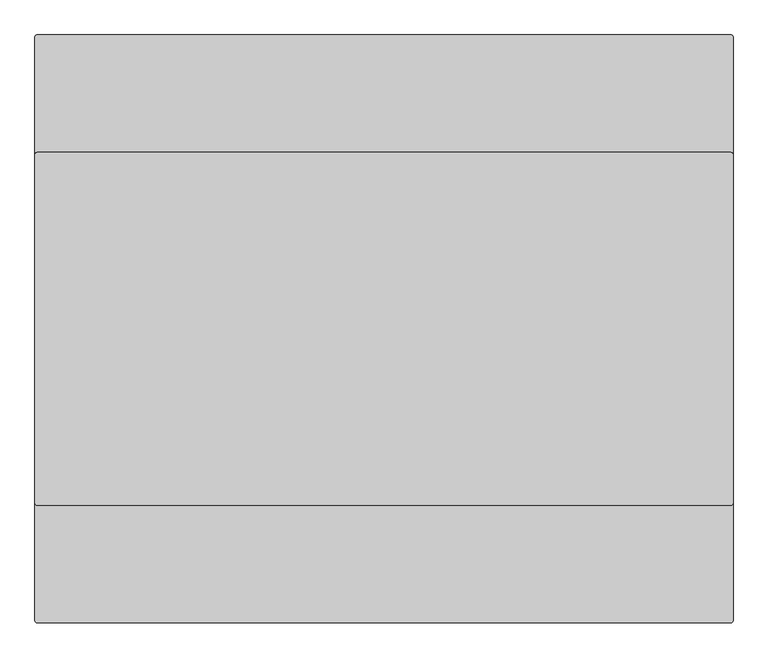
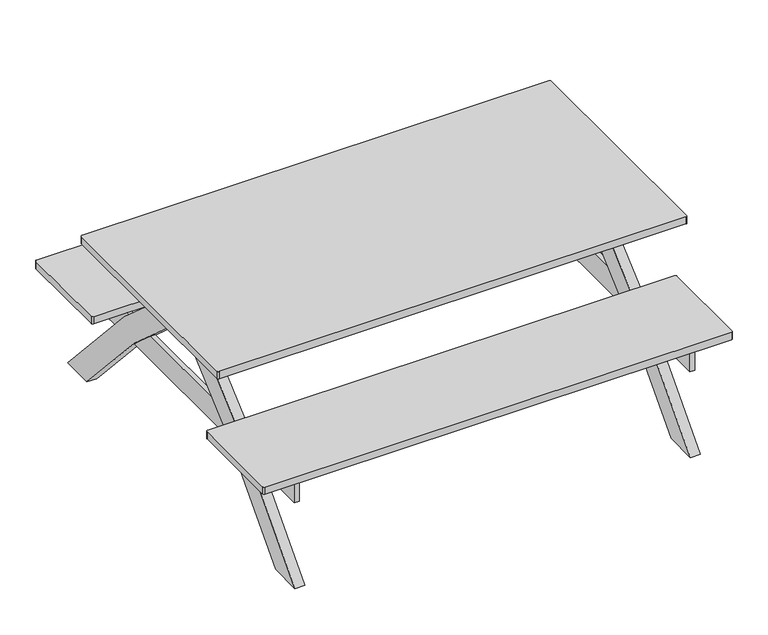
"""IFC4 building model written with IfcOpenShell, lengths in millimetres: furniture geometry, NLRS_90_FU_WPB_picknick tafel_gen_rsf : picknicktafel hout lxbxh 1900x1600x750mm."""

import ifcopenshell
import ifcopenshell.guid

model = None  # the IFC model being written
_history = None  # IfcOwnerHistory: only IFC2X3 demands one
_inside = {}  # id of a spatial element -> (the spatial element, [elements in it])
_under = {}  # id of a project, library or spatial element -> (it, [spatial elements below it])
_declared = {}  # id of a project -> (the project, [libraries it declares])
_typed = {}  # id of a type object -> (the type object, [elements of that type])
_made_of = {}  # id of a material, layer set ... -> (it, [elements and type objects made of it])


def new_model(schema):
    """Start an empty IFC model of exactly this schema.

    Asked for "IFC4X3", IfcOpenShell would pick the latest addendum, in which some entities
    have other attributes; the version numbers below select the first issue.
    IFC2X3 requires an IfcOwnerHistory on every rooted entity: one is made here for all.
    """
    global model, _history
    if schema == "IFC4X3":
        model = ifcopenshell.file(schema_version=(4, 3, 0, 0))
    else:
        model = ifcopenshell.file(schema=schema)
    _inside.clear()
    _under.clear()
    _declared.clear()
    _typed.clear()
    _made_of.clear()
    _history = None
    if model.schema == "IFC2X3":
        org = make("IfcOrganization", Name="unknown")
        user = make(
            "IfcPersonAndOrganization",
            ThePerson=make("IfcPerson", FamilyName="unknown"),
            TheOrganization=org,
        )
        app = make(
            "IfcApplication",
            ApplicationDeveloper=org,
            Version="unknown",
            ApplicationFullName="unknown",
            ApplicationIdentifier="unknown",
        )
        _history = make(
            "IfcOwnerHistory",
            OwningUser=user,
            OwningApplication=app,
            ChangeAction="ADDED",
            CreationDate=0,
        )
    return model


def make(cls, **values):
    """One entity of the class cls with the attributes given. An attribute that is None is left unset."""
    return model.create_entity(
        cls, **{name: value for name, value in values.items() if value is not None}
    )


def rooted(cls, **values):
    """An entity with a GlobalId (a new one), such as an element, a storey or a relation."""
    return make(cls, GlobalId=ifcopenshell.guid.new(), OwnerHistory=_history, **values)


def si_unit(unit_type, name, prefix=None):
    """IfcSIUnit, for example si_unit("LENGTHUNIT", "METRE", prefix="MILLI")."""
    return make("IfcSIUnit", UnitType=unit_type, Prefix=prefix, Name=name)


def assignment(units):
    """IfcUnitAssignment: the units of a project."""
    return None if units is None else make("IfcUnitAssignment", Units=units)


def point(xyz):
    """IfcCartesianPoint."""
    return None if xyz is None else make("IfcCartesianPoint", Coordinates=xyz)


def direction(xyz):
    """IfcDirection."""
    return None if xyz is None else make("IfcDirection", DirectionRatios=xyz)


def frame(location, z_axis=None, x_axis=None):
    """IfcAxis2Placement3D, a coordinate frame: its origin and axes. An axis left out is left unset."""
    return make(
        "IfcAxis2Placement3D",
        Location=point(location),
        Axis=direction(z_axis),
        RefDirection=direction(x_axis),
    )


def frame_2d(location, x_axis=None):
    """IfcAxis2Placement2D, a coordinate frame in the plane: its origin and x axis."""
    return make(
        "IfcAxis2Placement2D", Location=point(location), RefDirection=direction(x_axis)
    )


def origin():
    """The frame at (0, 0, 0) with its axes left unset."""
    return frame((0.0, 0.0, 0.0))


def place(relative_to, where):
    """IfcLocalPlacement: puts the frame where relative to a parent placement (None: the world)."""
    return make(
        "IfcLocalPlacement", PlacementRelTo=relative_to, RelativePlacement=where
    )


def context(
    kind, dimensions, precision=None, world=None, true_north=None, identifier=None
):
    """IfcGeometricRepresentationContext, for example the 3D "Model" context."""
    return make(
        "IfcGeometricRepresentationContext",
        ContextIdentifier=identifier,
        ContextType=kind,
        CoordinateSpaceDimension=dimensions,
        Precision=precision,
        WorldCoordinateSystem=world,
        TrueNorth=true_north,
    )


def project(units=None, contexts=None):
    """IfcProject with its units and contexts."""
    return rooted(
        "IfcProject",
        Name="project",
        RepresentationContexts=contexts,
        UnitsInContext=assignment(units),
    )


def spatial(cls, under=None, at=None, **own):
    """A site, building, storey or space (cls), placed at a placement, below another one or the project."""
    s = rooted(cls, ObjectPlacement=at, **own)
    if under is not None:
        _under.setdefault(under.id(), (under, []))[1].append(s)
    return s


def polyline(points):
    """IfcPolyline through the points."""
    return make("IfcPolyline", Points=[point(p) for p in points])


def circle_curve(where, radius):
    """IfcCircle in the frame where."""
    return make("IfcCircle", Position=where, Radius=radius)


def trimmed(basis, trim1, trim2, sense, master):
    """IfcTrimmedCurve: the piece of a basis curve between two trims."""
    return make(
        "IfcTrimmedCurve",
        BasisCurve=basis,
        Trim1=trim1,
        Trim2=trim2,
        SenseAgreement=sense,
        MasterRepresentation=master,
    )


def segment(curve, same_sense, transition):
    """IfcCompositeCurveSegment."""
    return make(
        "IfcCompositeCurveSegment",
        Transition=transition,
        SameSense=same_sense,
        ParentCurve=curve,
    )


def composite_curve(segments, self_intersect=None):
    """IfcCompositeCurve: segments joined end to end."""
    return make("IfcCompositeCurve", Segments=segments, SelfIntersect=self_intersect)


def outline(outer, holes=None, kind="AREA"):
    """IfcArbitraryClosedProfileDef: a profile drawn as a closed curve; with holes, ...WithVoids."""
    if holes is None:
        return make("IfcArbitraryClosedProfileDef", ProfileType=kind, OuterCurve=outer)
    return make(
        "IfcArbitraryProfileDefWithVoids",
        ProfileType=kind,
        OuterCurve=outer,
        InnerCurves=holes,
    )


def extrude(swept, where, along, depth):
    """IfcExtrudedAreaSolid: the profile swept, set in the frame where, extruded along a direction by depth."""
    return make(
        "IfcExtrudedAreaSolid",
        SweptArea=swept,
        Position=where,
        ExtrudedDirection=direction(along),
        Depth=depth,
    )


def faces_of(points, faces, orient=None, outer=None):
    """IfcFace entities. A face is a list of loops; a loop is a list of indices into points, from 0.

    orient and outer hold one flag for each loop. By default every Orientation is true, the
    first loop of a face is its IfcFaceOuterBound and the others are IfcFaceBound.
    """
    made = []
    for i, loops in enumerate(faces):
        bounds = []
        for j, loop in enumerate(loops):
            is_outer = j == 0 if outer is None else outer[i][j]
            bounds.append(
                make(
                    "IfcFaceOuterBound" if is_outer else "IfcFaceBound",
                    Bound=make("IfcPolyLoop", Polygon=[points[k] for k in loop]),
                    Orientation=True if orient is None else orient[i][j],
                )
            )
        made.append(make("IfcFace", Bounds=bounds))
    return made


def faceted_brep(points, faces, orient=None, outer=None, voids=None):
    """IfcFacetedBrep: a solid bounded by flat faces; with voids (closed shells), ...WithVoids."""
    shared = [point(p) for p in points]
    hull = make("IfcClosedShell", CfsFaces=faces_of(shared, faces, orient, outer))
    if voids is None:
        return make("IfcFacetedBrep", Outer=hull)
    return make(
        "IfcFacetedBrepWithVoids",
        Outer=hull,
        Voids=[
            make(cls, CfsFaces=faces_of(shared, fs, o, b)) for cls, fs, o, b in voids
        ],
    )


def shape(context_of_items, identifier, shape_type, items):
    """IfcShapeRepresentation: the items that make up one representation, for example the "Body"."""
    return make(
        "IfcShapeRepresentation",
        ContextOfItems=context_of_items,
        RepresentationIdentifier=identifier,
        RepresentationType=shape_type,
        Items=items,
    )


def source(mapping_origin, context_of_items, identifier, shape_type, items):
    """IfcRepresentationMap: a shape defined once, which mapped items show again and again."""
    return make(
        "IfcRepresentationMap",
        MappingOrigin=mapping_origin,
        MappedRepresentation=shape(context_of_items, identifier, shape_type, items),
    )


def transform(
    local_origin,
    x_axis=None,
    y_axis=None,
    z_axis=None,
    scale=None,
    scale2=None,
    scale3=None,
    uniform=True,
):
    """IfcCartesianTransformationOperator3D, or its non-uniform kind. x_axis, y_axis, z_axis: its Axis1, 2, 3."""
    if uniform:
        return make(
            "IfcCartesianTransformationOperator3D",
            Axis1=direction(x_axis),
            Axis2=direction(y_axis),
            LocalOrigin=point(local_origin),
            Scale=scale,
            Axis3=direction(z_axis),
        )
    return make(
        "IfcCartesianTransformationOperator3DnonUniform",
        Axis1=direction(x_axis),
        Axis2=direction(y_axis),
        LocalOrigin=point(local_origin),
        Scale=scale,
        Axis3=direction(z_axis),
        Scale2=scale2,
        Scale3=scale3,
    )


def mapped(mapping_source, mapping_target):
    """IfcMappedItem: shows the shape of a source again, moved by a transform."""
    return make(
        "IfcMappedItem", MappingSource=mapping_source, MappingTarget=mapping_target
    )


def made_of(thing, what):
    """Note that an element or type object is made of a material, layer set ...; save() writes the relation."""
    if what is not None:
        _made_of.setdefault(what.id(), (what, []))[1].append(thing)
    return thing


def element(
    cls,
    number,
    at=None,
    inside=None,
    cuts=None,
    type_object=None,
    material=None,
    context=None,
    identifier="Body",
    shape_type=None,
    held_by="IfcProductDefinitionShape",
    body=None,
    shapes=None,
    **own,
):
    """One element of the class cls, such as IfcWall. Its Tag is "e" and its number.

    at: its placement. inside: the storey or other place that contains it. cuts: it is an
    opening in that element (IfcRelVoidsElement). A single representation is given by context,
    identifier, shape_type and body (its items); several are given by shapes. held_by: the class
    of the entity that holds the representations. save() writes the other relations.
    """
    e = rooted(cls, Tag="e%d" % number, ObjectPlacement=at, **own)
    if body is not None:
        shapes = [shape(context, identifier, shape_type, body)]
    if shapes is not None:
        e.Representation = make(held_by, Representations=shapes)
    if inside is not None:
        _inside.setdefault(inside.id(), (inside, []))[1].append(e)
    if cuts is not None:
        rooted(
            "IfcRelVoidsElement", RelatingBuildingElement=cuts, RelatedOpeningElement=e
        )
    if type_object is not None:
        _typed.setdefault(type_object.id(), (type_object, []))[1].append(e)
    return made_of(e, material)


def aggregate(whole, parts):
    """IfcRelAggregates: a whole, such as a stair, and the parts it consists of."""
    return rooted("IfcRelAggregates", RelatingObject=whole, RelatedObjects=parts)


def save(model, path):
    """Write the relations noted so far, then the file.

    IfcRelAggregates (storeys below a building ...), IfcRelContainedInSpatialStructure (elements
    in a storey), IfcRelDefinesByType, IfcRelAssociatesMaterial and IfcRelDeclares: one each for
    every whole, place, type object, material and project.
    """
    for whole, parts in _under.values():
        aggregate(whole, parts)
    for where, things in _inside.values():
        rooted(
            "IfcRelContainedInSpatialStructure",
            RelatedElements=things,
            RelatingStructure=where,
        )
    for kind, things in _typed.values():
        rooted("IfcRelDefinesByType", RelatedObjects=things, RelatingType=kind)
    for what, things in _made_of.values():
        rooted("IfcRelAssociatesMaterial", RelatedObjects=things, RelatingMaterial=what)
    for by, libraries in _declared.values():
        rooted("IfcRelDeclares", RelatingContext=by, RelatedDefinitions=libraries)
    model.write(path)


def furniture_9bce7ad1(model_context):
    return source(origin(), model_context, "Body", "SolidModel", [
        extrude(outline(composite_curve([segment(trimmed(circle_curve(frame_2d((943.65, 473.65)), 6.35), [point((943.65, 480.0))], [point((950.0, 473.65))], False, "CARTESIAN"), True, "CONTINUOUS"), segment(polyline([(950.0, 473.65), (950.0, -473.65)]), True, "CONTINUOUS"), segment(trimmed(circle_curve(frame_2d((943.65, -473.65)), 6.35), [point((950.0, -473.65))], [point((943.65, -480.0))], False, "CARTESIAN"), True, "CONTINUOUS"), segment(polyline([(943.65, -480.0), (-943.65, -480.0)]), True, "CONTINUOUS"), segment(trimmed(circle_curve(frame_2d((-943.65, -473.65)), 6.35), [point((-943.65, -480.0))], [point((-950.0, -473.65))], False, "CARTESIAN"), True, "CONTINUOUS"), segment(polyline([(-950.0, -473.65), (-950.0, 473.65)]), True, "CONTINUOUS"), segment(trimmed(circle_curve(frame_2d((-943.65, 473.65)), 6.35), [point((-950.0, 473.65))], [point((-943.65, 480.0))], False, "CARTESIAN"), True, "CONTINUOUS"), segment(polyline([(-943.65, 480.0), (943.65, 480.0)]), True, "CONTINUOUS")], self_intersect=False)), frame((0.0, 0.0, 750.0), z_axis=(0.0, 0.0, 1.0), x_axis=(1.0, 0.0, 0.0)), (0.0, 0.0, 1.0), 30.0),
        extrude(outline(composite_curve([segment(trimmed(circle_curve(frame_2d((943.65, -406.35)), 6.35), [point((943.65, -400.0))], [point((950.0, -406.35))], False, "CARTESIAN"), True, "CONTINUOUS"), segment(polyline([(950.0, -406.35), (950.0, -793.65)]), True, "CONTINUOUS"), segment(trimmed(circle_curve(frame_2d((943.65, -793.65)), 6.35), [point((950.0, -793.65))], [point((943.65, -800.0))], False, "CARTESIAN"), True, "CONTINUOUS"), segment(polyline([(943.65, -800.0), (-943.65, -800.0)]), True, "CONTINUOUS"), segment(trimmed(circle_curve(frame_2d((-943.65, -793.65)), 6.35), [point((-943.65, -800.0))], [point((-950.0, -793.65))], False, "CARTESIAN"), True, "CONTINUOUS"), segment(polyline([(-950.0, -793.65), (-950.0, -406.35)]), True, "CONTINUOUS"), segment(trimmed(circle_curve(frame_2d((-943.65, -406.35)), 6.35), [point((-950.0, -406.35))], [point((-943.65, -400.0))], False, "CARTESIAN"), True, "CONTINUOUS"), segment(polyline([(-943.65, -400.0), (943.65, -400.0)]), True, "CONTINUOUS")], self_intersect=False)), frame((0.0, 0.0, 450.0), z_axis=(0.0, 0.0, 1.0), x_axis=(1.0, 0.0, 0.0)), (0.0, 0.0, 1.0), 30.0),
        extrude(outline(composite_curve([segment(polyline([(943.65, 400.0), (-943.65, 400.0)]), True, "CONTINUOUS"), segment(trimmed(circle_curve(frame_2d((-943.65, 406.35)), 6.35), [point((-943.65, 400.0))], [point((-950.0, 406.35))], False, "CARTESIAN"), True, "CONTINUOUS"), segment(polyline([(-950.0, 406.35), (-950.0, 793.65)]), True, "CONTINUOUS"), segment(trimmed(circle_curve(frame_2d((-943.65, 793.65)), 6.35), [point((-950.0, 793.65))], [point((-943.65, 800.0))], False, "CARTESIAN"), True, "CONTINUOUS"), segment(polyline([(-943.65, 800.0), (943.65, 800.0)]), True, "CONTINUOUS"), segment(trimmed(circle_curve(frame_2d((943.65, 793.65)), 6.35), [point((943.65, 800.0))], [point((950.0, 793.65))], False, "CARTESIAN"), True, "CONTINUOUS"), segment(polyline([(950.0, 793.65), (950.0, 406.35)]), True, "CONTINUOUS"), segment(trimmed(circle_curve(frame_2d((943.65, 406.35)), 6.35), [point((950.0, 406.35))], [point((943.65, 400.0))], False, "CARTESIAN"), True, "CONTINUOUS")], self_intersect=False)), frame((0.0, 0.0, 450.0), z_axis=(0.0, 0.0, 1.0), x_axis=(1.0, 0.0, 0.0)), (0.0, 0.0, 1.0), 30.0),
        extrude(outline(polyline([(-790.0, 774.6), (-790.0, -774.6), (-810.0, -774.6), (-810.0, 774.6), (-790.0, 774.6)])), frame((0.0, 0.0, 350.0), z_axis=(0.0, 0.0, 1.0), x_axis=(1.0, 0.0, 0.0)), (0.0, 0.0, 1.0), 100.0),
        faceted_brep([(780.0, 47.1187461, 750.0), (780.0, 400.0, 437.3), (780.0, 795.7416498, 0.0), (780.0, 660.8726936, 0.0), (780.0, 329.5529767, 366.1128726), (780.0, 1.6260502, 656.7), (780.0, -1.6260502, 656.7), (780.0, -329.5529767, 366.1128726), (780.0, -660.8726936, 0.0), (780.0, -795.7416498, 0.0), (780.0, -400.0, 437.3), (780.0, -47.1187461, 750.0), (820.0, 47.1187461, 750.0), (820.0, -47.1187461, 750.0), (820.0, -400.0, 437.3), (820.0, -795.7416498, 0.0), (820.0, -660.8726936, 0.0), (820.0, -329.5529767, 366.1128726), (820.0, -1.6260502, 656.7), (820.0, 1.6260502, 656.7), (820.0, 329.5529767, 366.1128726), (820.0, 660.8726936, 0.0), (820.0, 795.7416498, 0.0), (820.0, 400.0, 437.3), (810.0, 400.0, 437.3), (810.0, 385.6680783, 450.0), (790.0, 385.6680783, 450.0), (790.0, 400.0, 437.3), (790.0, 479.0035354, 350.0), (810.0, 479.0035354, 350.0), (810.0, 329.5529767, 366.1128726), (810.0, 344.1345792, 350.0), (790.0, 344.1345792, 350.0), (790.0, 329.5529767, 366.1128726), (790.0, 234.8865401, 450.0), (810.0, 234.8865401, 450.0), (810.0, -329.5529767, 366.1128726), (810.0, -234.8865401, 450.0), (790.0, -234.8865401, 450.0), (790.0, -329.5529767, 366.1128726), (790.0, -344.1345792, 350.0), (810.0, -344.1345792, 350.0), (810.0, -400.0, 437.3), (810.0, -479.0035354, 350.0), (790.0, -479.0035354, 350.0), (790.0, -400.0, 437.3), (790.0, -385.6680783, 450.0), (810.0, -385.6680783, 450.0), (790.0, 774.6, 450.0), (790.0, 774.6, 350.0), (790.0, -774.6, 350.0), (790.0, -774.6, 450.0), (810.0, -774.6, 450.0), (810.0, -774.6, 350.0), (810.0, 774.6, 350.0), (810.0, 774.6, 450.0)], [[[0, 1, 2, 3, 4, 5, 6, 7, 8, 9, 10, 11]], [[12, 13, 14, 15, 16, 17, 18, 19, 20, 21, 22, 23]], [[1, 0, 12, 23, 24, 25, 26, 27]], [[2, 1, 27, 28, 29, 24, 23, 22]], [[3, 2, 22, 21]], [[4, 3, 21, 20, 30, 31, 32, 33]], [[5, 4, 33, 34, 35, 30, 20, 19]], [[6, 5, 19, 18]], [[7, 6, 18, 17, 36, 37, 38, 39]], [[8, 7, 39, 40, 41, 36, 17, 16]], [[9, 8, 16, 15]], [[10, 9, 15, 14, 42, 43, 44, 45]], [[11, 10, 45, 46, 47, 42, 14, 13]], [[0, 11, 13, 12]], [[48, 49, 28, 27, 26]], [[50, 51, 46, 45, 44]], [[38, 34, 33, 32, 40, 39]], [[52, 53, 43, 42, 47]], [[54, 55, 25, 24, 29]], [[41, 31, 30, 35, 37, 36]], [[37, 35, 34, 38]], [[51, 52, 47, 46]], [[55, 48, 26, 25]], [[49, 48, 55, 54]], [[31, 41, 40, 32]], [[49, 54, 29, 28]], [[53, 50, 44, 43]], [[51, 50, 53, 52]]]),
        extrude(outline(polyline([(47.1187461, 750.0), (400.0, 437.3), (795.7416498, 0.0), (660.8726936, 0.0), (329.5529767, 366.1128726), (1.6260502, 656.7), (-1.6260502, 656.7), (-329.5529767, 366.1128726), (-660.8726936, 0.0), (-795.7416498, 0.0), (-400.0, 437.3), (-47.1187461, 750.0), (47.1187461, 750.0)])), frame((-820.0, 0.0, 0.0), z_axis=(1.0, 0.0, 0.0), x_axis=(0.0, 1.0, 0.0)), (0.0, 0.0, 1.0), 40.0),
    ])


if __name__ == "__main__":
    model = new_model("IFC4")
    model_context = context("Model", 3, world=origin())
    ifc_project = project(units=[si_unit("LENGTHUNIT", "METRE", prefix="MILLI")], contexts=[model_context])
    site = spatial("IfcSite", under=ifc_project)
    building = spatial("IfcBuilding", under=site)
    placement = place(None, origin())
    furniture_shape = furniture_9bce7ad1(model_context)
    element("IfcFurniture", 1, ObjectType="NLRS_90_FU_WPB_picknick tafel_gen_rsf : picknicktafel hout lxbxh 1900x1600x750mm", at=placement, inside=building, context=model_context, shape_type="MappedRepresentation", body=[
        mapped(furniture_shape, transform((0.0, 0.0, 0.0), x_axis=(1.0, 0.0, 0.0), y_axis=(0.0, 1.0, 0.0), z_axis=(0.0, 0.0, 1.0))),
    ])
    save(model, "model.ifc")

# Revit data of these elements
# Type "NLRS_90_FU_WPB_picknick tafel_gen_rsf : picknicktafel hout lxbxh 1900x1600x750mm"
#   Type IfcGUID = "05J6pyYiTDtR2exmlhyPT4"
#   IfcName[Type] = "picknicktafel hout lxbxh 1900x1600x750mm"
#   IfcDescription[Type] = "picknicktafel hout lxbxh 1900x1600x750mm"
#   IfcObjectType[Type] = "TABLE"
#   IfcExportAs[Type] = "IfcGeographicElementType"
#   IfcExportType[Type] = "USERDEFINED"
#   NLRS_C_omschrijving_02 [instance default] = "zitbank"
#   NLRS_C_omschrijving_01 [instance default] = "tafelblad"
#   NLRS_C_revit_versie = ""
#   NLRS_C_content_versie = ""
#   NLRS_C_content_provider = ""
#   NLRS_C_content_handleiding = ""
#   NLRS_C_content_datum_uitgifte = ""
#   NLRS_C_content_datum_gewijzigd = ""
#   NLRS_C_content_creator = ""
#   Model = "generiek"
#   Manufacturer = "Revit Standards Foundation"
#   Description = "picknicktafel hout lxbxh 1900x1600x750mm"
#   Assembly Code = "90.71"
#   bf_overstek = 150.00 mm
#   NLRS_C_hoogte_01 = 450.00 mm
#   NLRS_C_hoogte = 750.00 mm
#   NLRS_C_dikte_02 = 30.00 mm
#   NLRS_C_dikte_01 = 30.00 mm
#   NLRS_C_diepte_02 = 960.00 mm
#   NLRS_C_diepte_01 = 400.00 mm
#   NLRS_C_diepte = 1600.00 mm
#   NLRS_C_breedte = 1900.00 mm
#   Default Elevation = 1219.20 mm
#   NLRS_C_materiaal_02 = NLRS_i3_hout loofhout meranti vernis planken 120mm_gen_rsf
#   NLRS_C_materiaal_01 = NLRS_i3_hout loofhout meranti vernis planken 120mm_gen_rsf
#   NLRS_C_materiaal = NLRS_i3_hout loofhout meranti vernis_gen_rsf
# Element 1 (IfcFurniture, "NLRS_90_FU_WPB_picknick tafel_gen_rsf : picknicktafel hout lxbxh 1900x1600x750mm")
#   Materials on its faces: "NLRS_i3_hout loofhout meranti vernis_gen_rsf", "NLRS_i3_hout loofhout meranti vernis planken 120mm_gen_rsf"
# Materials
#   "NLRS_i3_hout loofhout meranti vernis planken 120mm_gen_rsf": class "Unassigned", colour RGB 227 170 128, transparency 0, Keynote = "i3", Model = "generiek", Manufacturer = "Revit Standards Foundation", URL = "www.revitstandards.org", Description = "loofhout merantie vernis planken 120mm", Cost = 0
#   "NLRS_i3_hout loofhout meranti vernis_gen_rsf": class "Unassigned", colour RGB 227 170 128, transparency 0, Keynote = "i3", Model = "generiek", Manufacturer = "Revit Standards Foundation", URL = "www.revitstandards.org", Description = "loofhout merantie vernis", Cost = 0
